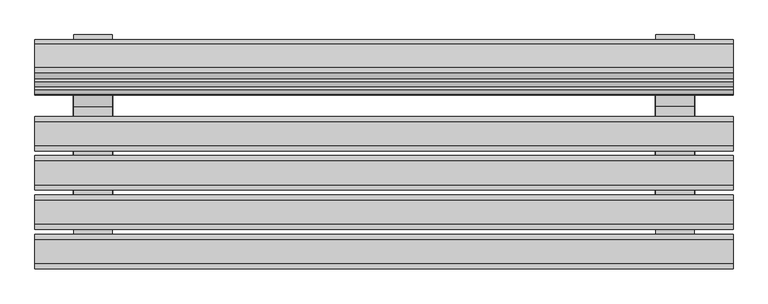
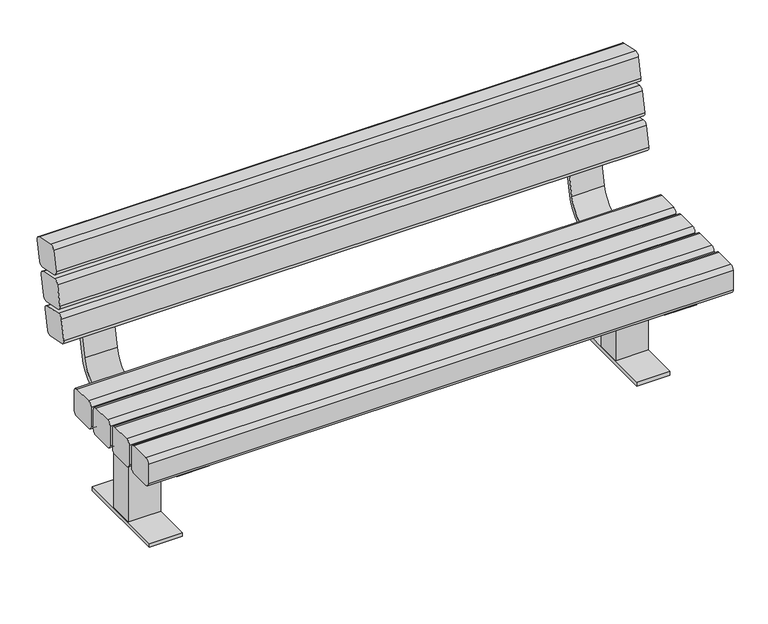
"""IFC4 building model written with IfcOpenShell, lengths in millimetres: furniture geometry, NLRS_90_FU_WPB_parkbank_gen_rsf : 1800mm breed."""

from ifc_helpers import new_model, si_unit, point, frame, frame_2d, origin, origin_with_axes, place, context, project, spatial, polyline, circle_curve, trimmed, segment, composite_curve, outline, extrude, source, transform, mapped, element, save


def furniture_f8362c1b(model_context):
    return source(origin(), model_context, "Body", "SweptSolid", [
        extrude(outline(polyline([(-778.4316018, -207.3631555), (-676.8316018, -207.3631555), (-676.8316018, -512.1631555), (-778.4316018, -512.1631555), (-778.4316018, -207.3631555)])), origin_with_axes(), (0.0, 0.0, 1.0), 12.7),
        extrude(outline(polyline([(722.3683982, -321.6631555), (822.3683982, -321.6631555), (822.3683982, -397.8631555), (722.3683982, -397.8631555), (722.3683982, -321.6631555)])), frame((0.0, 0.0, 12.7), z_axis=(0.0, 0.0, 1.0), x_axis=(1.0, 0.0, 0.0)), (0.0, 0.0, 1.0), 304.8),
        extrude(outline(composite_curve([segment(polyline([(-85.9429731, 777.6296037), (-73.5204986, 774.9891252), (-152.5879669, 403.005933)]), True, "CONTINUOUS"), segment(trimmed(circle_curve(frame_2d((-258.1790004, 425.45)), 107.95), [point((-152.5879669, 403.005933))], [point((-258.1790004, 317.5))], False, "CARTESIAN"), True, "CONTINUOUS"), segment(polyline([(-258.1790004, 317.5), (-656.6612098, 317.5), (-656.6612098, 330.1516727), (-258.1892727, 330.1516727)]), True, "CONTINUOUS"), segment(trimmed(circle_curve(frame_2d((-258.1892727, 425.4016727)), 95.25), [point((-258.1892727, 330.1516727))], [point((-165.0207138, 405.5980841))], True, "CARTESIAN"), True, "CONTINUOUS"), segment(polyline([(-165.0207138, 405.5980841), (-85.9429731, 777.6296037)]), True, "CONTINUOUS")], self_intersect=False)), frame((722.3683982, 0.0, 0.0), z_axis=(1.0, 0.0, 0.0), x_axis=(0.0, 1.0, 0.0)), (0.0, 0.0, 1.0), 100.0),
        extrude(outline(polyline([(-677.6316018, -321.6631555), (-677.6316018, -397.8631555), (-777.6316018, -397.8631555), (-777.6316018, -321.6631555), (-677.6316018, -321.6631555)])), frame((0.0, 0.0, 12.7), z_axis=(0.0, 0.0, 1.0), x_axis=(1.0, 0.0, 0.0)), (0.0, 0.0, 1.0), 304.8),
        extrude(outline(polyline([(823.1683982, -207.3631555), (823.1683982, -512.1631555), (721.5683982, -512.1631555), (721.5683982, -207.3631555), (823.1683982, -207.3631555)])), origin_with_axes(), (0.0, 0.0, 1.0), 12.7),
        extrude(outline(composite_curve([segment(polyline([(-200.0849974, 607.1353566), (-137.9726248, 593.9329642)]), True, "CONTINUOUS"), segment(trimmed(circle_curve(frame_2d((-140.6131032, 581.5104897)), 12.7), [point((-137.9726248, 593.9329642))], [point((-128.1906287, 578.8700112))], False, "CARTESIAN"), True, "CONTINUOUS"), segment(polyline([(-128.1906287, 578.8700112), (-141.3930211, 516.7576386)]), True, "CONTINUOUS"), segment(trimmed(circle_curve(frame_2d((-153.8154956, 519.398117)), 12.7), [point((-141.3930211, 516.7576386))], [point((-156.4559741, 506.9756425))], False, "CARTESIAN"), True, "CONTINUOUS"), segment(polyline([(-156.4559741, 506.9756425), (-218.5683467, 520.1780349)]), True, "CONTINUOUS"), segment(trimmed(circle_curve(frame_2d((-215.9278683, 532.6005094)), 12.7), [point((-218.5683467, 520.1780349))], [point((-228.3503428, 535.2409879))], False, "CARTESIAN"), True, "CONTINUOUS"), segment(polyline([(-228.3503428, 535.2409879), (-215.1479504, 597.3533605)]), True, "CONTINUOUS"), segment(trimmed(circle_curve(frame_2d((-202.7254759, 594.7128821)), 12.7), [point((-215.1479504, 597.3533605))], [point((-200.0849974, 607.1353566))], False, "CARTESIAN"), True, "CONTINUOUS")], self_intersect=False)), frame((-877.6316018, 0.0, 0.0), z_axis=(1.0, 0.0, 0.0), x_axis=(0.0, 1.0, 0.0)), (0.0, 0.0, 1.0), 1800.0),
        extrude(outline(composite_curve([segment(polyline([(-178.9611696, 706.5151528), (-116.848797, 693.3127605)]), True, "CONTINUOUS"), segment(trimmed(circle_curve(frame_2d((-119.4892755, 680.8902859)), 12.7), [point((-116.848797, 693.3127605))], [point((-107.0668009, 678.2498075))], False, "CARTESIAN"), True, "CONTINUOUS"), segment(polyline([(-107.0668009, 678.2498075), (-120.2691933, 616.1374348)]), True, "CONTINUOUS"), segment(trimmed(circle_curve(frame_2d((-132.6916678, 618.7779133)), 12.7), [point((-120.2691933, 616.1374348))], [point((-135.3321463, 606.3554388))], False, "CARTESIAN"), True, "CONTINUOUS"), segment(polyline([(-135.3321463, 606.3554388), (-197.4445189, 619.5578311)]), True, "CONTINUOUS"), segment(trimmed(circle_curve(frame_2d((-194.8040405, 631.9803056)), 12.7), [point((-197.4445189, 619.5578311))], [point((-207.226515, 634.6207841))], False, "CARTESIAN"), True, "CONTINUOUS"), segment(polyline([(-207.226515, 634.6207841), (-194.0241226, 696.7331568)]), True, "CONTINUOUS"), segment(trimmed(circle_curve(frame_2d((-181.6016481, 694.0926783)), 12.7), [point((-194.0241226, 696.7331568))], [point((-178.9611696, 706.5151528))], False, "CARTESIAN"), True, "CONTINUOUS")], self_intersect=False)), frame((-877.6316018, 0.0, 0.0), z_axis=(1.0, 0.0, 0.0), x_axis=(0.0, 1.0, 0.0)), (0.0, 0.0, 1.0), 1800.0),
        extrude(outline(composite_curve([segment(polyline([(-85.9429731, 777.6296037), (-73.5204986, 774.9891252), (-152.5879669, 403.005933)]), True, "CONTINUOUS"), segment(trimmed(circle_curve(frame_2d((-258.1790004, 425.45)), 107.95), [point((-152.5879669, 403.005933))], [point((-258.1790004, 317.5))], False, "CARTESIAN"), True, "CONTINUOUS"), segment(polyline([(-258.1790004, 317.5), (-656.6612098, 317.5), (-656.6612098, 330.1516727), (-258.1892727, 330.1516727)]), True, "CONTINUOUS"), segment(trimmed(circle_curve(frame_2d((-258.1892727, 425.4016727)), 95.25), [point((-258.1892727, 330.1516727))], [point((-165.0207138, 405.5980841))], True, "CARTESIAN"), True, "CONTINUOUS"), segment(polyline([(-165.0207138, 405.5980841), (-85.9429731, 777.6296037)]), True, "CONTINUOUS")], self_intersect=False)), frame((-777.6316018, 0.0, 0.0), z_axis=(1.0, 0.0, 0.0), x_axis=(0.0, 1.0, 0.0)), (0.0, 0.0, 1.0), 100.0),
        extrude(outline(composite_curve([segment(polyline([(-157.8373418, 805.8949491), (-95.7249692, 792.6925567)]), True, "CONTINUOUS"), segment(trimmed(circle_curve(frame_2d((-98.3654477, 780.2700822)), 12.7), [point((-95.7249692, 792.6925567))], [point((-85.9429731, 777.6296037))], False, "CARTESIAN"), True, "CONTINUOUS"), segment(polyline([(-85.9429731, 777.6296037), (-99.1453655, 715.517231)]), True, "CONTINUOUS"), segment(trimmed(circle_curve(frame_2d((-111.56784, 718.1577095)), 12.7), [point((-99.1453655, 715.517231))], [point((-114.2083185, 705.735235))], False, "CARTESIAN"), True, "CONTINUOUS"), segment(polyline([(-114.2083185, 705.735235), (-176.3206912, 718.9376274)]), True, "CONTINUOUS"), segment(trimmed(circle_curve(frame_2d((-173.6802127, 731.3601019)), 12.7), [point((-176.3206912, 718.9376274))], [point((-186.1026872, 734.0005804))], False, "CARTESIAN"), True, "CONTINUOUS"), segment(polyline([(-186.1026872, 734.0005804), (-172.9002948, 796.112953)]), True, "CONTINUOUS"), segment(trimmed(circle_curve(frame_2d((-160.4778203, 793.4724745)), 12.7), [point((-172.9002948, 796.112953))], [point((-157.8373418, 805.8949491))], False, "CARTESIAN"), True, "CONTINUOUS")], self_intersect=False)), frame((-877.6316018, 0.0, 0.0), z_axis=(1.0, 0.0, 0.0), x_axis=(0.0, 1.0, 0.0)), (0.0, 0.0, 1.0), 1800.0),
        extrude(outline(composite_curve([segment(polyline([(-665.0298429, 419.0516727), (-601.5298429, 419.0516727)]), True, "CONTINUOUS"), segment(trimmed(circle_curve(frame_2d((-601.5298429, 406.3516727)), 12.7), [point((-601.5298429, 419.0516727))], [point((-588.8298429, 406.3516727))], False, "CARTESIAN"), True, "CONTINUOUS"), segment(polyline([(-588.8298429, 406.3516727), (-588.8298429, 342.8516727)]), True, "CONTINUOUS"), segment(trimmed(circle_curve(frame_2d((-601.5298429, 342.8516727)), 12.7), [point((-588.8298429, 342.8516727))], [point((-601.5298429, 330.1516727))], False, "CARTESIAN"), True, "CONTINUOUS"), segment(polyline([(-601.5298429, 330.1516727), (-665.0298429, 330.1516727)]), True, "CONTINUOUS"), segment(trimmed(circle_curve(frame_2d((-665.0298429, 342.8516727)), 12.7), [point((-665.0298429, 330.1516727))], [point((-677.7298429, 342.8516727))], False, "CARTESIAN"), True, "CONTINUOUS"), segment(polyline([(-677.7298429, 342.8516727), (-677.7298429, 406.3516727)]), True, "CONTINUOUS"), segment(trimmed(circle_curve(frame_2d((-665.0298429, 406.3516727)), 12.7), [point((-677.7298429, 406.3516727))], [point((-665.0298429, 419.0516727))], False, "CARTESIAN"), True, "CONTINUOUS")], self_intersect=False)), frame((-877.6316018, 0.0, 0.0), z_axis=(1.0, 0.0, 0.0), x_axis=(0.0, 1.0, 0.0)), (0.0, 0.0, 1.0), 1800.0),
        extrude(outline(composite_curve([segment(polyline([(-563.4298429, 419.0516727), (-499.9298429, 419.0516727)]), True, "CONTINUOUS"), segment(trimmed(circle_curve(frame_2d((-499.9298429, 406.3516727)), 12.7), [point((-499.9298429, 419.0516727))], [point((-487.2298429, 406.3516727))], False, "CARTESIAN"), True, "CONTINUOUS"), segment(polyline([(-487.2298429, 406.3516727), (-487.2298429, 342.8516727)]), True, "CONTINUOUS"), segment(trimmed(circle_curve(frame_2d((-499.9298429, 342.8516727)), 12.7), [point((-487.2298429, 342.8516727))], [point((-499.9298429, 330.1516727))], False, "CARTESIAN"), True, "CONTINUOUS"), segment(polyline([(-499.9298429, 330.1516727), (-563.4298429, 330.1516727)]), True, "CONTINUOUS"), segment(trimmed(circle_curve(frame_2d((-563.4298429, 342.8516727)), 12.7), [point((-563.4298429, 330.1516727))], [point((-576.1298429, 342.8516727))], False, "CARTESIAN"), True, "CONTINUOUS"), segment(polyline([(-576.1298429, 342.8516727), (-576.1298429, 406.3516727)]), True, "CONTINUOUS"), segment(trimmed(circle_curve(frame_2d((-563.4298429, 406.3516727)), 12.7), [point((-576.1298429, 406.3516727))], [point((-563.4298429, 419.0516727))], False, "CARTESIAN"), True, "CONTINUOUS")], self_intersect=False)), frame((-877.6316018, 0.0, 0.0), z_axis=(1.0, 0.0, 0.0), x_axis=(0.0, 1.0, 0.0)), (0.0, 0.0, 1.0), 1800.0),
        extrude(outline(composite_curve([segment(polyline([(-461.8298429, 419.0516727), (-398.3298429, 419.0516727)]), True, "CONTINUOUS"), segment(trimmed(circle_curve(frame_2d((-398.3298429, 406.3516727)), 12.7), [point((-398.3298429, 419.0516727))], [point((-385.6298429, 406.3516727))], False, "CARTESIAN"), True, "CONTINUOUS"), segment(polyline([(-385.6298429, 406.3516727), (-385.6298429, 342.8516727)]), True, "CONTINUOUS"), segment(trimmed(circle_curve(frame_2d((-398.3298429, 342.8516727)), 12.7), [point((-385.6298429, 342.8516727))], [point((-398.3298429, 330.1516727))], False, "CARTESIAN"), True, "CONTINUOUS"), segment(polyline([(-398.3298429, 330.1516727), (-461.8298429, 330.1516727)]), True, "CONTINUOUS"), segment(trimmed(circle_curve(frame_2d((-461.8298429, 342.8516727)), 12.7), [point((-461.8298429, 330.1516727))], [point((-474.5298429, 342.8516727))], False, "CARTESIAN"), True, "CONTINUOUS"), segment(polyline([(-474.5298429, 342.8516727), (-474.5298429, 406.3516727)]), True, "CONTINUOUS"), segment(trimmed(circle_curve(frame_2d((-461.8298429, 406.3516727)), 12.7), [point((-474.5298429, 406.3516727))], [point((-461.8298429, 419.0516727))], False, "CARTESIAN"), True, "CONTINUOUS")], self_intersect=False)), frame((-877.6316018, 0.0, 0.0), z_axis=(1.0, 0.0, 0.0), x_axis=(0.0, 1.0, 0.0)), (0.0, 0.0, 1.0), 1800.0),
        extrude(outline(composite_curve([segment(polyline([(-360.2298429, 419.0516727), (-296.7298429, 419.0516727)]), True, "CONTINUOUS"), segment(trimmed(circle_curve(frame_2d((-296.7298429, 406.3516727)), 12.7), [point((-296.7298429, 419.0516727))], [point((-284.0298429, 406.3516727))], False, "CARTESIAN"), True, "CONTINUOUS"), segment(polyline([(-284.0298429, 406.3516727), (-284.0298429, 342.8516727)]), True, "CONTINUOUS"), segment(trimmed(circle_curve(frame_2d((-296.7298429, 342.8516727)), 12.7), [point((-284.0298429, 342.8516727))], [point((-296.7298429, 330.1516727))], False, "CARTESIAN"), True, "CONTINUOUS"), segment(polyline([(-296.7298429, 330.1516727), (-360.2298429, 330.1516727)]), True, "CONTINUOUS"), segment(trimmed(circle_curve(frame_2d((-360.2298429, 342.8516727)), 12.7), [point((-360.2298429, 330.1516727))], [point((-372.9298429, 342.8516727))], False, "CARTESIAN"), True, "CONTINUOUS"), segment(polyline([(-372.9298429, 342.8516727), (-372.9298429, 406.3516727)]), True, "CONTINUOUS"), segment(trimmed(circle_curve(frame_2d((-360.2298429, 406.3516727)), 12.7), [point((-372.9298429, 406.3516727))], [point((-360.2298429, 419.0516727))], False, "CARTESIAN"), True, "CONTINUOUS")], self_intersect=False)), frame((-877.6316018, 0.0, 0.0), z_axis=(1.0, 0.0, 0.0), x_axis=(0.0, 1.0, 0.0)), (0.0, 0.0, 1.0), 1800.0),
    ])


if __name__ == "__main__":
    model = new_model("IFC4")
    model_context = context("Model", 3, world=origin())
    ifc_project = project(units=[si_unit("LENGTHUNIT", "METRE", prefix="MILLI")], contexts=[model_context])
    site = spatial("IfcSite", under=ifc_project)
    building = spatial("IfcBuilding", under=site)
    placement = place(None, origin())
    furniture_shape = furniture_f8362c1b(model_context)
    element("IfcFurniture", 1, ObjectType="NLRS_90_FU_WPB_parkbank_gen_rsf : 1800mm breed", at=placement, inside=building, context=model_context, shape_type="MappedRepresentation", body=[
        mapped(furniture_shape, transform((0.0, 0.0, 0.0), x_axis=(1.0, 0.0, 0.0), y_axis=(0.0, 1.0, 0.0), z_axis=(0.0, 0.0, 1.0))),
    ])
    save(model, "model.ifc")

# Revit data of these elements
# Type "NLRS_90_FU_WPB_parkbank_gen_rsf : 1800mm breed"
#   Type IFC Predefined Type = "USERDEFINED"
#   Export Type to IFC As = "IfcGeographicElementType"
#   Type IfcGUID = "05J6pyYiTDtR2exmlhyPly"
#   IfcName[Type] = "parkbank 1800mm breed"
#   IfcDescription[Type] = "parkbank b 1800mm"
#   IfcObjectType[Type] = "BENCH"
#   NLRS_C_revit_versie = ""
#   NLRS_C_omschrijving_02 = "onderstel"
#   NLRS_C_omschrijving_01 = "zitting"
#   NLRS_C_content_versie = ""
#   NLRS_C_content_provider = ""
#   NLRS_C_content_handleiding = ""
#   NLRS_C_content_datum_uitgifte = ""
#   NLRS_C_content_datum_gewijzigd = ""
#   NLRS_C_content_creator = ""
#   Model = "generiek"
#   Manufacturer = "Revit Standards Foundation"
#   Description = "parkbank b 1800mm"
#   Assembly Code = "90.71"
#   bf_overstek = 150.00 mm
#   NLRS_C_hoogte_01 [instance default] = 419.052 mm
#   NLRS_C_hoogte [instance default] = 806.45 mm
#   NLRS_C_diepte_01 [instance default] = 372.631 mm
#   NLRS_C_breedte = 1800.00 mm
#   Default Elevation = 1219.20 mm
#   NLRS_C_materiaal_02 = NLRS_h2_staal mat gepolijst grijs_gen_rsf
#   NLRS_C_materiaal_01 = NLRS_i3_hout loofhout meranti vernis_gen_rsf
# Element 1 (IfcFurniture, "NLRS_90_FU_WPB_parkbank_gen_rsf : 1800mm breed")
#   Materials on its faces: "NLRS_i3_hout loofhout meranti vernis_gen_rsf", "NLRS_h2_staal mat gepolijst grijs_gen_rsf"
# Materials
#   "NLRS_h2_staal mat gepolijst grijs_gen_rsf": class "System", colour RGB 189 187 185, transparency 0, Keynote = "h2", Model = "generiek", Manufacturer = "Revit Standards Foundation", URL = "www.revitstandards.org", Description = "staal mat gepolijst", Cost = 0
#   "NLRS_i3_hout loofhout meranti vernis_gen_rsf": class "Unassigned", colour RGB 227 170 128, transparency 0, Keynote = "i3", Model = "generiek", Manufacturer = "Revit Standards Foundation", URL = "www.revitstandards.org", Description = "loofhout merantie vernis", Cost = 0
